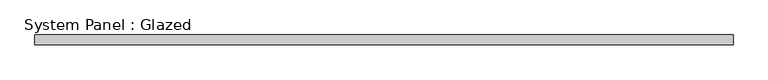
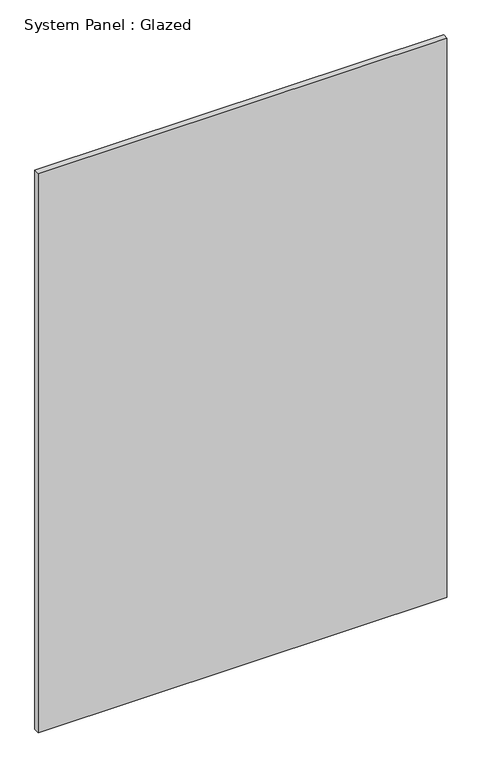
"""IFC4 building model written with IfcOpenShell, lengths in millimetres: plate geometry, System Panel : Glazed."""

from ifc_helpers import new_model, si_unit, origin, origin_with_axes, place, context, project, spatial, polyline, outline, extrude, source, transform, mapped, element, save


def system_panel_glazed_fdadfa8c(model_context):
    return source(origin(), model_context, "Body", "SweptSolid", [
        extrude(outline(polyline([(906.9444446, 24.5), (-906.9444446, 24.5), (-906.9444446, 49.5), (906.9444446, 49.5), (906.9444446, 24.5)])), origin_with_axes(), (0.0, 0.0, 1.0), 2625.0),
    ])


if __name__ == "__main__":
    model = new_model("IFC4")
    model_context = context("Model", 3, world=origin())
    ifc_project = project(units=[si_unit("LENGTHUNIT", "METRE", prefix="MILLI")], contexts=[model_context])
    site = spatial("IfcSite", under=ifc_project)
    building = spatial("IfcBuilding", under=site)
    placement = place(None, origin())
    system_panel_glazed_shape = system_panel_glazed_fdadfa8c(model_context)
    element("IfcPlate", 1, ObjectType="System Panel : Glazed", at=placement, inside=building, context=model_context, shape_type="MappedRepresentation", body=[
        mapped(system_panel_glazed_shape, transform((0.0, 0.0, 0.0), x_axis=(1.0, 0.0, 0.0), y_axis=(0.0, 1.0, 0.0), z_axis=(0.0, 0.0, 1.0))),
    ])
    save(model, "model.ifc")

# Revit data of these elements
# Element 1 (IfcPlate, "System Panel : Glazed")
#   Materials on its faces: "Glass"
# Materials
#   "Glass": class "Glass", colour RGB 0 128 192, transparency 0.9
